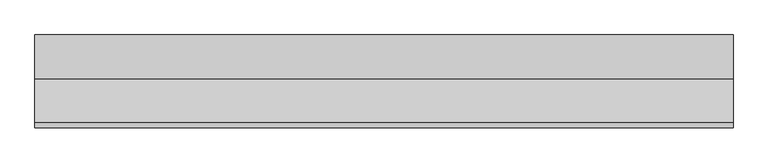
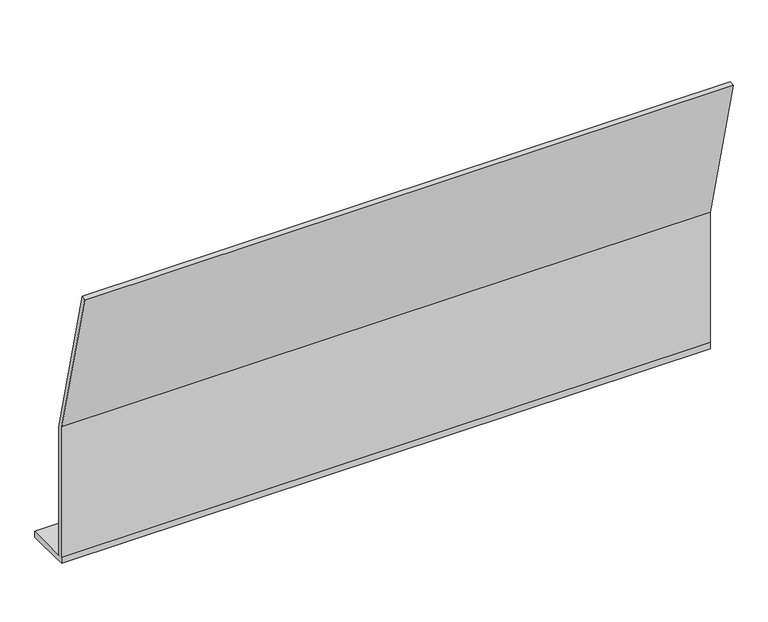
"""IFC4 building model written with IfcOpenShell, lengths in millimetres: proxy geometry, Gypsum016 3086 : Gypsum016 3086."""

import ifcopenshell
import ifcopenshell.guid

model = None  # the IFC model being written
_history = None  # IfcOwnerHistory: only IFC2X3 demands one
_inside = {}  # id of a spatial element -> (the spatial element, [elements in it])
_under = {}  # id of a project, library or spatial element -> (it, [spatial elements below it])
_declared = {}  # id of a project -> (the project, [libraries it declares])
_typed = {}  # id of a type object -> (the type object, [elements of that type])
_made_of = {}  # id of a material, layer set ... -> (it, [elements and type objects made of it])


def new_model(schema):
    """Start an empty IFC model of exactly this schema.

    Asked for "IFC4X3", IfcOpenShell would pick the latest addendum, in which some entities
    have other attributes; the version numbers below select the first issue.
    IFC2X3 requires an IfcOwnerHistory on every rooted entity: one is made here for all.
    """
    global model, _history
    if schema == "IFC4X3":
        model = ifcopenshell.file(schema_version=(4, 3, 0, 0))
    else:
        model = ifcopenshell.file(schema=schema)
    _inside.clear()
    _under.clear()
    _declared.clear()
    _typed.clear()
    _made_of.clear()
    _history = None
    if model.schema == "IFC2X3":
        org = make("IfcOrganization", Name="unknown")
        user = make(
            "IfcPersonAndOrganization",
            ThePerson=make("IfcPerson", FamilyName="unknown"),
            TheOrganization=org,
        )
        app = make(
            "IfcApplication",
            ApplicationDeveloper=org,
            Version="unknown",
            ApplicationFullName="unknown",
            ApplicationIdentifier="unknown",
        )
        _history = make(
            "IfcOwnerHistory",
            OwningUser=user,
            OwningApplication=app,
            ChangeAction="ADDED",
            CreationDate=0,
        )
    return model


def make(cls, **values):
    """One entity of the class cls with the attributes given. An attribute that is None is left unset."""
    return model.create_entity(
        cls, **{name: value for name, value in values.items() if value is not None}
    )


def rooted(cls, **values):
    """An entity with a GlobalId (a new one), such as an element, a storey or a relation."""
    return make(cls, GlobalId=ifcopenshell.guid.new(), OwnerHistory=_history, **values)


def si_unit(unit_type, name, prefix=None):
    """IfcSIUnit, for example si_unit("LENGTHUNIT", "METRE", prefix="MILLI")."""
    return make("IfcSIUnit", UnitType=unit_type, Prefix=prefix, Name=name)


def assignment(units):
    """IfcUnitAssignment: the units of a project."""
    return None if units is None else make("IfcUnitAssignment", Units=units)


def point(xyz):
    """IfcCartesianPoint."""
    return None if xyz is None else make("IfcCartesianPoint", Coordinates=xyz)


def direction(xyz):
    """IfcDirection."""
    return None if xyz is None else make("IfcDirection", DirectionRatios=xyz)


def frame(location, z_axis=None, x_axis=None):
    """IfcAxis2Placement3D, a coordinate frame: its origin and axes. An axis left out is left unset."""
    return make(
        "IfcAxis2Placement3D",
        Location=point(location),
        Axis=direction(z_axis),
        RefDirection=direction(x_axis),
    )


def origin():
    """The frame at (0, 0, 0) with its axes left unset."""
    return frame((0.0, 0.0, 0.0))


def place(relative_to, where):
    """IfcLocalPlacement: puts the frame where relative to a parent placement (None: the world)."""
    return make(
        "IfcLocalPlacement", PlacementRelTo=relative_to, RelativePlacement=where
    )


def context(
    kind, dimensions, precision=None, world=None, true_north=None, identifier=None
):
    """IfcGeometricRepresentationContext, for example the 3D "Model" context."""
    return make(
        "IfcGeometricRepresentationContext",
        ContextIdentifier=identifier,
        ContextType=kind,
        CoordinateSpaceDimension=dimensions,
        Precision=precision,
        WorldCoordinateSystem=world,
        TrueNorth=true_north,
    )


def project(units=None, contexts=None):
    """IfcProject with its units and contexts."""
    return rooted(
        "IfcProject",
        Name="project",
        RepresentationContexts=contexts,
        UnitsInContext=assignment(units),
    )


def spatial(cls, under=None, at=None, **own):
    """A site, building, storey or space (cls), placed at a placement, below another one or the project."""
    s = rooted(cls, ObjectPlacement=at, **own)
    if under is not None:
        _under.setdefault(under.id(), (under, []))[1].append(s)
    return s


def polyline(points):
    """IfcPolyline through the points."""
    return make("IfcPolyline", Points=[point(p) for p in points])


def outline(outer, holes=None, kind="AREA"):
    """IfcArbitraryClosedProfileDef: a profile drawn as a closed curve; with holes, ...WithVoids."""
    if holes is None:
        return make("IfcArbitraryClosedProfileDef", ProfileType=kind, OuterCurve=outer)
    return make(
        "IfcArbitraryProfileDefWithVoids",
        ProfileType=kind,
        OuterCurve=outer,
        InnerCurves=holes,
    )


def extrude(swept, where, along, depth):
    """IfcExtrudedAreaSolid: the profile swept, set in the frame where, extruded along a direction by depth."""
    return make(
        "IfcExtrudedAreaSolid",
        SweptArea=swept,
        Position=where,
        ExtrudedDirection=direction(along),
        Depth=depth,
    )


def shape(context_of_items, identifier, shape_type, items):
    """IfcShapeRepresentation: the items that make up one representation, for example the "Body"."""
    return make(
        "IfcShapeRepresentation",
        ContextOfItems=context_of_items,
        RepresentationIdentifier=identifier,
        RepresentationType=shape_type,
        Items=items,
    )


def source(mapping_origin, context_of_items, identifier, shape_type, items):
    """IfcRepresentationMap: a shape defined once, which mapped items show again and again."""
    return make(
        "IfcRepresentationMap",
        MappingOrigin=mapping_origin,
        MappedRepresentation=shape(context_of_items, identifier, shape_type, items),
    )


def transform(
    local_origin,
    x_axis=None,
    y_axis=None,
    z_axis=None,
    scale=None,
    scale2=None,
    scale3=None,
    uniform=True,
):
    """IfcCartesianTransformationOperator3D, or its non-uniform kind. x_axis, y_axis, z_axis: its Axis1, 2, 3."""
    if uniform:
        return make(
            "IfcCartesianTransformationOperator3D",
            Axis1=direction(x_axis),
            Axis2=direction(y_axis),
            LocalOrigin=point(local_origin),
            Scale=scale,
            Axis3=direction(z_axis),
        )
    return make(
        "IfcCartesianTransformationOperator3DnonUniform",
        Axis1=direction(x_axis),
        Axis2=direction(y_axis),
        LocalOrigin=point(local_origin),
        Scale=scale,
        Axis3=direction(z_axis),
        Scale2=scale2,
        Scale3=scale3,
    )


def mapped(mapping_source, mapping_target):
    """IfcMappedItem: shows the shape of a source again, moved by a transform."""
    return make(
        "IfcMappedItem", MappingSource=mapping_source, MappingTarget=mapping_target
    )


def made_of(thing, what):
    """Note that an element or type object is made of a material, layer set ...; save() writes the relation."""
    if what is not None:
        _made_of.setdefault(what.id(), (what, []))[1].append(thing)
    return thing


def element(
    cls,
    number,
    at=None,
    inside=None,
    cuts=None,
    type_object=None,
    material=None,
    context=None,
    identifier="Body",
    shape_type=None,
    held_by="IfcProductDefinitionShape",
    body=None,
    shapes=None,
    **own,
):
    """One element of the class cls, such as IfcWall. Its Tag is "e" and its number.

    at: its placement. inside: the storey or other place that contains it. cuts: it is an
    opening in that element (IfcRelVoidsElement). A single representation is given by context,
    identifier, shape_type and body (its items); several are given by shapes. held_by: the class
    of the entity that holds the representations. save() writes the other relations.
    """
    e = rooted(cls, Tag="e%d" % number, ObjectPlacement=at, **own)
    if body is not None:
        shapes = [shape(context, identifier, shape_type, body)]
    if shapes is not None:
        e.Representation = make(held_by, Representations=shapes)
    if inside is not None:
        _inside.setdefault(inside.id(), (inside, []))[1].append(e)
    if cuts is not None:
        rooted(
            "IfcRelVoidsElement", RelatingBuildingElement=cuts, RelatedOpeningElement=e
        )
    if type_object is not None:
        _typed.setdefault(type_object.id(), (type_object, []))[1].append(e)
    return made_of(e, material)


def aggregate(whole, parts):
    """IfcRelAggregates: a whole, such as a stair, and the parts it consists of."""
    return rooted("IfcRelAggregates", RelatingObject=whole, RelatedObjects=parts)


def save(model, path):
    """Write the relations noted so far, then the file.

    IfcRelAggregates (storeys below a building ...), IfcRelContainedInSpatialStructure (elements
    in a storey), IfcRelDefinesByType, IfcRelAssociatesMaterial and IfcRelDeclares: one each for
    every whole, place, type object, material and project.
    """
    for whole, parts in _under.values():
        aggregate(whole, parts)
    for where, things in _inside.values():
        rooted(
            "IfcRelContainedInSpatialStructure",
            RelatedElements=things,
            RelatingStructure=where,
        )
    for kind, things in _typed.values():
        rooted("IfcRelDefinesByType", RelatedObjects=things, RelatingType=kind)
    for what, things in _made_of.values():
        rooted("IfcRelAssociatesMaterial", RelatedObjects=things, RelatingMaterial=what)
    for by, libraries in _declared.values():
        rooted("IfcRelDeclares", RelatingContext=by, RelatedDefinitions=libraries)
    model.write(path)


def generic_models_b19d98fa(model_context):
    return source(origin(), model_context, "Body", "SweptSolid", [
        extrude(outline(polyline([(10404.7574604, 42887.9921875), (10283.0402569, 42887.9921875), (10283.0402569, 42889.2721875), (10261.8870729, 42889.2721875), (10261.8870729, 42910.4253714), (10260.6070729, 42910.4253714), (10260.6070729, 43334.9453125), (10138.6847483, 43822.1948052), (10152.7950131, 43825.7223714), (10278.0250834, 43324.8020904), (10278.0250834, 42906.696), (10404.7574604, 42906.696), (10404.7574604, 42887.9921875)])), frame((3694.2883192, 0.0, 0.0), z_axis=(1.0, 0.0, 0.0), x_axis=(0.0, 1.0, 0.0)), (0.0, 0.0, 1.0), 2000.0),
    ])


if __name__ == "__main__":
    model = new_model("IFC4")
    model_context = context("Model", 3, world=origin())
    ifc_project = project(units=[si_unit("LENGTHUNIT", "METRE", prefix="MILLI")], contexts=[model_context])
    site = spatial("IfcSite", under=ifc_project)
    building = spatial("IfcBuilding", under=site)
    placement = place(None, origin())
    generic_models_shape = generic_models_b19d98fa(model_context)
    element("IfcBuildingElementProxy", 1, Name="Gypsum016 3086 : Gypsum016 3086", ObjectType="Gypsum016 3086 : Gypsum016 3086", at=placement, inside=building, context=model_context, shape_type="MappedRepresentation", body=[
        mapped(generic_models_shape, transform((0.0, 0.0, 0.0), x_axis=(1.0, 0.0, 0.0), y_axis=(0.0, 1.0, 0.0), z_axis=(0.0, 0.0, 1.0))),
    ])
    save(model, "model.ifc")

# Revit data of these elements
# Type "Gypsum016 3086 : Gypsum016 3086"
#   NameOverride = "Gypsum016"
# Element 1 (IfcBuildingElementProxy, "Gypsum016 3086 : Gypsum016 3086")
#   Materials on its faces: "5/8\"  GYPSUM BOARD"
# Materials
#   "5/8\"  GYPSUM BOARD": class "Unassigned", colour RGB 255 255 255, transparency 0, Cost = 0
